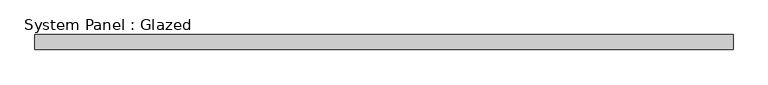
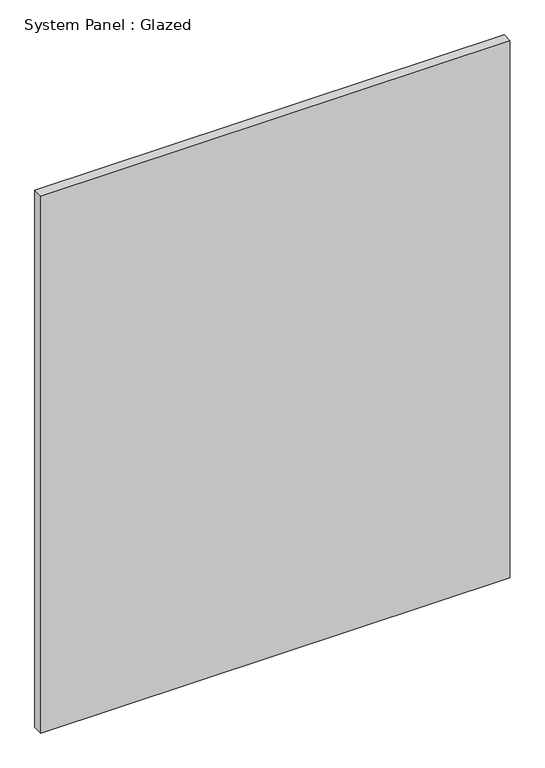
"""IFC4 building model written with IfcOpenShell, lengths in millimetres: plate geometry, System Panel : Glazed."""

from ifc_helpers import new_model, si_unit, origin, origin_with_axes, place, context, project, spatial, polyline, outline, extrude, source, transform, mapped, element, save


def system_panel_glazed_7324ab11(model_context):
    return source(origin(), model_context, "Body", "SweptSolid", [
        extrude(outline(polyline([(579.1666667, 24.5), (-579.1666667, 24.5), (-579.1666667, 49.5), (579.1666667, 49.5), (579.1666667, 24.5)])), origin_with_axes(), (0.0, 0.0, 1.0), 1400.0),
    ])


if __name__ == "__main__":
    model = new_model("IFC4")
    model_context = context("Model", 3, world=origin())
    ifc_project = project(units=[si_unit("LENGTHUNIT", "METRE", prefix="MILLI")], contexts=[model_context])
    site = spatial("IfcSite", under=ifc_project)
    building = spatial("IfcBuilding", under=site)
    placement = place(None, origin())
    system_panel_glazed_shape = system_panel_glazed_7324ab11(model_context)
    element("IfcPlate", 1, ObjectType="System Panel : Glazed", at=placement, inside=building, context=model_context, shape_type="MappedRepresentation", body=[
        mapped(system_panel_glazed_shape, transform((0.0, 0.0, 0.0), x_axis=(1.0, 0.0, 0.0), y_axis=(0.0, 1.0, 0.0), z_axis=(0.0, 0.0, 1.0))),
    ])
    save(model, "model.ifc")

# Revit data of these elements
# Element 1 (IfcPlate, "System Panel : Glazed")
#   Materials on its faces: "Glass"
# Materials
#   "Glass": class "Glass", colour RGB 0 128 192, transparency 0.9
